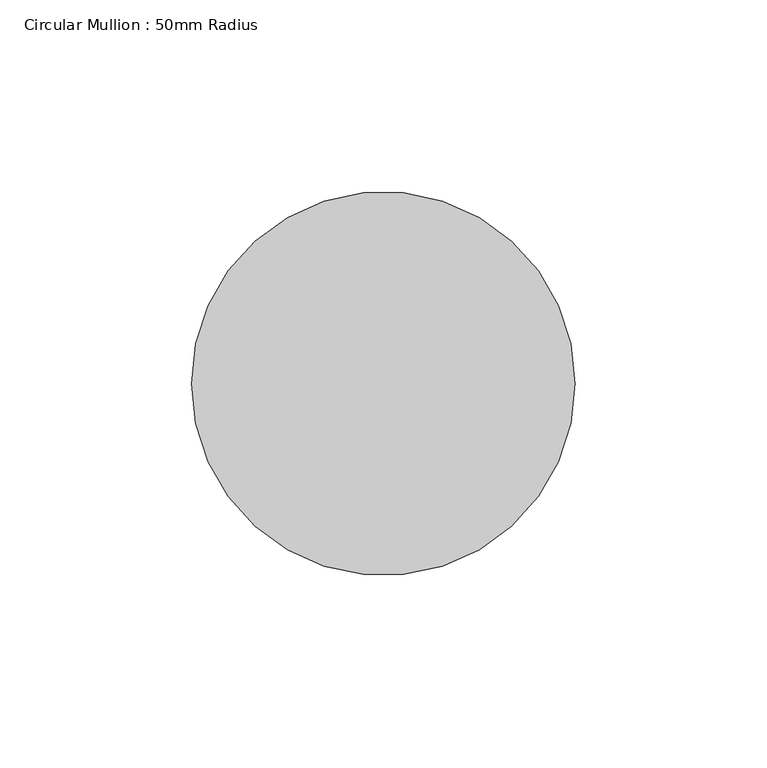
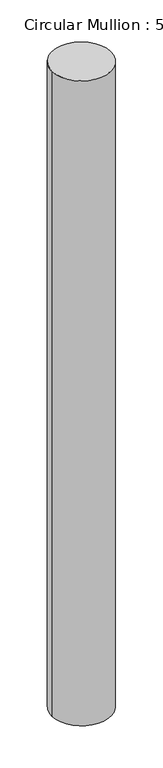
"""IFC4 building model written with IfcOpenShell, lengths in millimetres: member geometry, Circular Mullion : 50mm Radius."""

from ifc_helpers import new_model, si_unit, point, frame, origin, origin_2d, place, context, project, spatial, circle_curve, trimmed, segment, composite_curve, outline, extrude, source, transform, mapped, element, save


def circular_mullion_50mm_radius_22a54a8e(model_context):
    return source(origin(), model_context, "Body", "SweptSolid", [
        extrude(outline(composite_curve([segment(trimmed(circle_curve(origin_2d(), 50.0), [point((50.0, 0.0))], [point((-50.0, 0.0))], False, "CARTESIAN"), True, "CONTINUOUS"), segment(trimmed(circle_curve(origin_2d(), 50.0), [point((-50.0, 0.0))], [point((50.0, 0.0))], False, "CARTESIAN"), True, "CONTINUOUS")], self_intersect=False)), frame((0.0, 0.0, -1159.465226), z_axis=(0.0, 0.0, 1.0), x_axis=(1.0, 0.0, 0.0)), (0.0, 0.0, 1.0), 1159.465226),
    ])


if __name__ == "__main__":
    model = new_model("IFC4")
    model_context = context("Model", 3, world=origin())
    ifc_project = project(units=[si_unit("LENGTHUNIT", "METRE", prefix="MILLI")], contexts=[model_context])
    site = spatial("IfcSite", under=ifc_project)
    building = spatial("IfcBuilding", under=site)
    placement = place(None, origin())
    circular_mullion_50mm_radius_shape = circular_mullion_50mm_radius_22a54a8e(model_context)
    element("IfcMember", 1, ObjectType="Circular Mullion : 50mm Radius", at=placement, inside=building, context=model_context, shape_type="MappedRepresentation", body=[
        mapped(circular_mullion_50mm_radius_shape, transform((0.0, 0.0, 0.0), x_axis=(1.0, 0.0, 0.0), y_axis=(0.0, 1.0, 0.0), z_axis=(0.0, 0.0, 1.0))),
    ])
    save(model, "model.ifc")

# Revit data of these elements
# Type "Circular Mullion : 50mm Radius"
#   built-in parameter 1007350 = 0.164042 (stored number, unit not read)
# Element 1 (IfcMember, "Circular Mullion : 50mm Radius")
#   Materials on its faces: "Aluminium"
# Materials
#   "Aluminium": class "Metal", colour RGB 247 247 247, transparency 0, Description = "Aluminium 6061", Cost = 0
